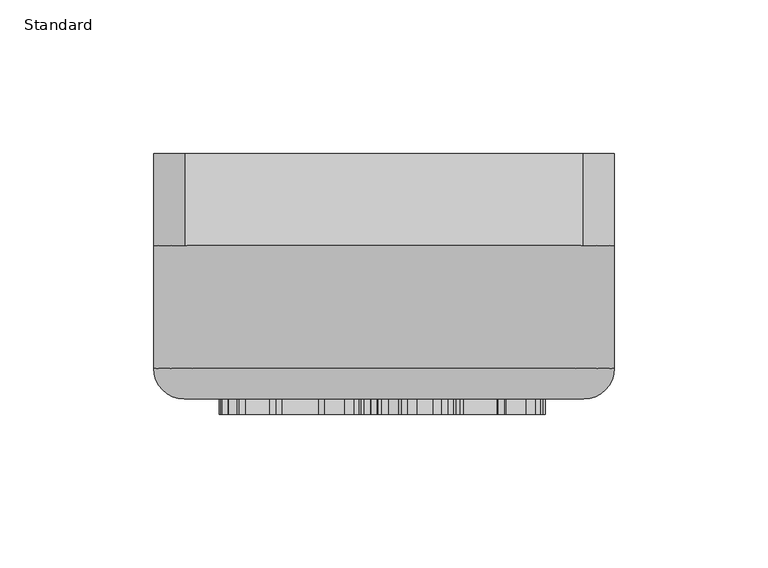
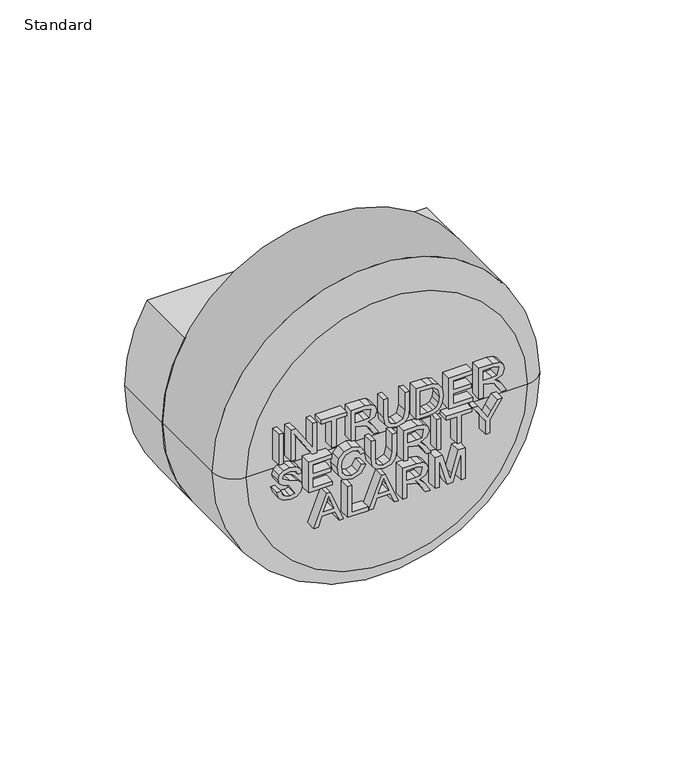
"""IFC4 building model written with IfcOpenShell, lengths in millimetres: proxy geometry, Intruder Security Alarm Sounder : Standard."""

from ifc_helpers import new_model, si_unit, point, frame, origin, origin_2d, place, context, project, spatial, polyline, circle_curve, ellipse_curve, trimmed, segment, composite_curve, outline, extrude, source, transform, mapped, element, save
from ifc_brep_helpers import plane_surface, cylinder_surface, revolved_surface, advanced_brep


def standard_da8f596e(model_context):
    return source(origin(), model_context, "Body", "SolidModel", [
        extrude(outline(polyline([(-50.8099209, -85.0), (-52.6934767, -85.0), (-52.6934767, -80.0), (-50.8099209, -80.0), (-50.8099209, -85.0)])), frame((0.0, 0.0, 4.6605901), z_axis=(0.0, 0.0, 1.0), x_axis=(1.0, 0.0, 0.0)), (0.0, 0.0, 1.0), 15.0684465),
        extrude(outline(polyline([(4.6605901, -47.0428093), (4.6605901, -45.1592535), (16.6020397, -45.1592535), (4.6605901, -37.2865788), (4.6605901, -35.2705855), (19.7290366, -35.2705855), (19.7290366, -37.1541413), (7.7912659, -37.1541413), (19.7290366, -45.026816), (19.7290366, -47.0428093), (4.6605901, -47.0428093)])), frame((0.0, -85.0, 0.0), z_axis=(0.0, 1.0, 0.0), x_axis=(0.0, 0.0, 1.0)), (0.0, 0.0, 1.0), 5.0),
        extrude(outline(polyline([(4.6605901, -28.2072512), (4.6605901, -26.3236953), (17.8454808, -26.3236953), (17.8454808, -21.3793613), (19.7290366, -21.3793613), (19.7290366, -33.1515852), (17.8454808, -33.1515852), (17.8454808, -28.2072512), (4.6605901, -28.2072512)])), frame((0.0, -85.0, 0.0), z_axis=(0.0, 1.0, 0.0), x_axis=(0.0, 0.0, 1.0)), (0.0, 0.0, 1.0), 5.0),
        extrude(outline(polyline([(4.6605901, -19.260361), (4.6605901, -17.3768052), (11.2530355, -17.3768052), (9.8514051, -12.1197715), (7.7839082, -10.7034258), (4.6605901, -8.7426148), (4.6605901, -6.5537169), (8.7440802, -9.0663509), (11.4884799, -11.6635978), (12.8901103, -8.5090097), (15.6050795, -7.4881372), (17.8841084, -8.1043395), (19.322527, -9.7524509), (19.7290366, -12.7672438), (19.7290366, -19.260361), (4.6605901, -19.260361)]), holes=[polyline([(13.1365913, -17.3768052), (17.8454808, -17.3768052), (17.8454808, -12.6863098), (17.1943297, -10.1681575), (13.4033057, -11.0106073), (13.1365913, -13.1608775), (13.1365913, -17.3768052)])]), frame((0.0, -85.0, 0.0), z_axis=(0.0, 1.0, 0.0), x_axis=(0.0, 0.0, 1.0)), (0.0, 0.0, 1.0), 5.0),
        extrude(outline(polyline([(19.7290366, 5.6967535), (11.1022038, 5.6967535), (7.298304, 4.7439392), (6.3087014, 1.5544023), (6.809021, -0.6602474), (8.2308849, -1.9367979), (11.1022038, -2.3083587), (19.7290366, -2.3083587), (19.7290366, -4.1919145), (11.0359851, -4.1919145), (7.2633552, -3.619858), (5.153552, -1.7105504), (4.4251456, 1.7309856), (5.2620772, 5.2258646), (7.4325809, 7.0689534), (11.0359851, 7.5803093), (19.7290366, 7.5803093), (19.7290366, 5.6967535)])), frame((0.0, -85.0, 0.0), z_axis=(0.0, 1.0, 0.0), x_axis=(0.0, 0.0, 1.0)), (0.0, 0.0, 1.0), 5.0),
        extrude(outline(polyline([(4.6605901, 10.876532), (4.6605901, 16.3248644), (4.9181075, 18.7473673), (5.674105, 20.5481497), (7.0407866, 21.9240283), (9.2352027, 22.9540979), (12.2757474, 23.3550893), (15.858918, 22.7627993), (18.434092, 20.9785716), (19.5119862, 18.763922), (19.7290366, 16.0747046), (19.7290366, 10.876532), (4.6605901, 10.876532)]), holes=[polyline([(6.5441459, 12.7600878), (17.8454808, 12.7600878), (17.8454808, 16.0415952), (17.5438176, 18.7124185), (15.8736333, 20.6677113), (12.305178, 21.4715335), (9.4559319, 21.0613451), (7.585252, 19.9153926), (6.8163786, 18.5174411), (6.5441459, 16.0930987), (6.5441459, 12.7600878)])]), frame((0.0, -85.0, 0.0), z_axis=(0.0, 1.0, 0.0), x_axis=(0.0, 0.0, 1.0)), (0.0, 0.0, 1.0), 5.0),
        extrude(outline(polyline([(4.6605901, 25.9449785), (4.6605901, 37.010869), (6.5441459, 37.010869), (6.5441459, 27.8285344), (11.4884799, 27.8285344), (11.4884799, 36.3045355), (13.3720357, 36.3045355), (13.3720357, 27.8285344), (17.8454808, 27.8285344), (17.8454808, 36.7754245), (19.7290366, 36.7754245), (19.7290366, 25.9449785), (4.6605901, 25.9449785)])), frame((0.0, -85.0, 0.0), z_axis=(0.0, 1.0, 0.0), x_axis=(0.0, 0.0, 1.0)), (0.0, 0.0, 1.0), 5.0),
        extrude(outline(polyline([(4.6605901, 39.8362027), (4.6605901, 41.7197585), (11.2530355, 41.7197585), (9.8514051, 46.9767922), (7.7839082, 48.3931379), (4.6605901, 50.3539489), (4.6605901, 52.5428468), (8.7440802, 50.0302128), (11.4884799, 47.4329659), (12.8901103, 50.587554), (15.6050795, 51.6084265), (17.8841084, 50.9922242), (19.322527, 49.3441128), (19.7290366, 46.3293199), (19.7290366, 39.8362027), (4.6605901, 39.8362027)]), holes=[polyline([(13.1365913, 41.7197585), (17.8454808, 41.7197585), (17.8454808, 46.4102539), (17.1943297, 48.9284062), (13.4033057, 48.0859564), (13.1365913, 45.9356862), (13.1365913, 41.7197585)])]), frame((0.0, -85.0, 0.0), z_axis=(0.0, 1.0, 0.0), x_axis=(0.0, 0.0, 1.0)), (0.0, 0.0, 1.0), 5.0),
        extrude(outline(polyline([(-8.4558541, -53.6352547), (-11.3326913, -52.8222354), (-13.23832, -50.6940381), (-13.8710771, -47.3297573), (-13.2843053, -44.4805112), (-11.6398728, -42.5380943), (-9.3865955, -41.8630308), (-7.2565588, -42.4498026), (-5.7298485, -44.2726579), (-4.7843918, -47.6056688), (-2.4262682, -51.2808099), (-0.8627697, -50.4346813), (-0.2152974, -47.7381063), (-0.8701273, -45.0488889), (-2.8051866, -43.9820311), (-2.8051866, -42.0984753), (-0.447063, -42.8452757), (1.1311507, -44.8318385), (1.6682584, -47.8116827), (1.155063, -50.603907), (-0.3495743, -52.5113752), (-2.4814505, -53.1643657), (-4.3539698, -52.636455), (-5.7556002, -51.034329), (-6.6845023, -48.0820759), (-11.6435516, -45.435165), (-11.9875212, -47.4033337), (-11.533187, -49.6621291), (-10.3412493, -51.1446935), (-8.4558541, -51.7516988), (-8.4558541, -53.6352547)])), frame((0.0, -85.0, 0.0), z_axis=(0.0, 1.0, 0.0), x_axis=(0.0, 0.0, 1.0)), (0.0, 0.0, 1.0), 5.0),
        extrude(outline(polyline([(-13.6356326, -39.0376971), (-13.6356326, -27.9718067), (-11.7520768, -27.9718067), (-11.7520768, -37.1541413), (-6.8077427, -37.1541413), (-6.8077427, -28.6781401), (-4.9241869, -28.6781401), (-4.9241869, -37.1541413), (-0.4507419, -37.1541413), (-0.4507419, -28.2072512), (1.4328139, -28.2072512), (1.4328139, -39.0376971), (-13.6356326, -39.0376971)])), frame((0.0, -85.0, 0.0), z_axis=(0.0, 1.0, 0.0), x_axis=(0.0, 0.0, 1.0)), (0.0, 0.0, 1.0), 5.0),
        extrude(outline(polyline([(-8.2792707, -14.5514715), (-11.053101, -16.1499188), (-11.9875212, -19.0322742), (-11.3014213, -21.6313605), (-9.2284063, -23.4008729), (-5.9836871, -23.9692506), (-3.1841051, -23.4891646), (-1.020959, -21.8244985), (-0.2152974, -18.8777638), (-0.9418643, -16.3320203), (-3.2576815, -14.786916), (-2.8088655, -12.9033602), (0.4947149, -15.0315575), (1.6682584, -18.8041874), (0.7614293, -22.4241462), (-1.8928393, -24.9606925), (-5.9873659, -25.8528064), (-10.0156737, -25.0636995), (-12.8814745, -22.764437), (-13.8710771, -18.8446544), (-12.5632566, -14.9009594), (-8.764875, -12.6679157), (-8.2792707, -14.5514715)])), frame((0.0, -85.0, 0.0), z_axis=(0.0, 1.0, 0.0), x_axis=(0.0, 0.0, 1.0)), (0.0, 0.0, 1.0), 5.0),
        extrude(outline(polyline([(1.4328139, -0.1893584), (-7.1940188, -0.1893584), (-10.9979187, -1.1421728), (-11.9875212, -4.3317097), (-11.4872017, -6.5463593), (-10.0653378, -7.8229098), (-7.1940188, -8.1944706), (1.4328139, -8.1944706), (1.4328139, -10.0780264), (-7.2602376, -10.0780264), (-11.0328675, -9.5059699), (-13.1426707, -7.5966624), (-13.8710771, -4.1551263), (-13.0341455, -0.6602474), (-10.8636417, 1.1828414), (-7.2602376, 1.6941974), (1.4328139, 1.6941974), (1.4328139, -0.1893584)])), frame((0.0, -85.0, 0.0), z_axis=(0.0, 1.0, 0.0), x_axis=(0.0, 0.0, 1.0)), (0.0, 0.0, 1.0), 5.0),
        extrude(outline(polyline([(-13.6356326, 4.9904201), (-13.6356326, 6.8739759), (-7.0431872, 6.8739759), (-8.4448176, 12.1310096), (-10.5123144, 13.5473553), (-13.6356326, 15.5081663), (-13.6356326, 17.6970642), (-9.5521424, 15.1844302), (-6.8077427, 12.5871833), (-5.4061123, 15.7417714), (-2.6911432, 16.7626439), (-0.4121143, 16.1464416), (1.0263043, 14.4983303), (1.4328139, 11.4835373), (1.4328139, 4.9904201), (-13.6356326, 4.9904201)]), holes=[polyline([(-5.1596314, 6.8739759), (-0.4507419, 6.8739759), (-0.4507419, 11.5644713), (-1.101893, 14.0826236), (-4.892917, 13.2401738), (-5.1596314, 11.0899036), (-5.1596314, 6.8739759)])]), frame((0.0, -85.0, 0.0), z_axis=(0.0, 1.0, 0.0), x_axis=(0.0, 0.0, 1.0)), (0.0, 0.0, 1.0), 5.0),
        extrude(outline(polyline([(22.1778669, -85.0), (20.2943111, -85.0), (20.2943111, -80.0), (22.1778669, -80.0), (22.1778669, -85.0)])), frame((0.0, 0.0, -13.6356326), z_axis=(0.0, 0.0, 1.0), x_axis=(1.0, 0.0, 0.0)), (0.0, 0.0, 1.0), 15.0684465),
        extrude(outline(polyline([(-13.6356326, 29.7120902), (-13.6356326, 31.595646), (-0.4507419, 31.595646), (-0.4507419, 36.53998), (1.4328139, 36.53998), (1.4328139, 24.7677562), (-0.4507419, 24.7677562), (-0.4507419, 29.7120902), (-13.6356326, 29.7120902)])), frame((0.0, -85.0, 0.0), z_axis=(0.0, 1.0, 0.0), x_axis=(0.0, 0.0, 1.0)), (0.0, 0.0, 1.0), 5.0),
        extrude(outline(polyline([(-13.6356326, 42.8969809), (-13.6356326, 44.7805367), (-7.25288, 44.7805367), (1.4328139, 50.6666486), (1.4328139, 48.4446414), (-3.0369523, 45.5935559), (-5.5716592, 43.9822328), (-3.206178, 42.3745884), (1.4328139, 39.2328762), (1.4328139, 37.010869), (-7.25288, 42.8969809), (-13.6356326, 42.8969809)])), frame((0.0, -85.0, 0.0), z_axis=(0.0, 1.0, 0.0), x_axis=(0.0, 0.0, 1.0)), (0.0, 0.0, 1.0), 5.0),
        extrude(outline(polyline([(-31.9318553, -36.5544936), (-31.9318553, -34.564252), (-27.2229657, -32.8425643), (-27.2229657, -26.636395), (-31.9318553, -24.9110285), (-31.9318553, -22.9207869), (-16.8634087, -28.9356575), (-16.8634087, -30.539623), (-31.9318553, -36.5544936)]), holes=[polyline([(-25.3394099, -32.1509461), (-21.3111021, -30.6757393), (-18.7469645, -29.7376403), (-21.6348382, -28.6818189), (-25.3394099, -27.3243344), (-25.3394099, -32.1509461)])]), frame((0.0, -85.0, 0.0), z_axis=(0.0, 1.0, 0.0), x_axis=(0.0, 0.0, 1.0)), (0.0, 0.0, 1.0), 5.0),
        extrude(outline(polyline([(-31.9318553, -20.9084724), (-31.9318553, -11.4906933), (-30.0482994, -11.4906933), (-30.0482994, -19.0249166), (-16.8634087, -19.0249166), (-16.8634087, -20.9084724), (-31.9318553, -20.9084724)])), frame((0.0, -85.0, 0.0), z_axis=(0.0, 1.0, 0.0), x_axis=(0.0, 0.0, 1.0)), (0.0, 0.0, 1.0), 5.0),
        extrude(outline(polyline([(-31.9318553, -11.1264901), (-31.9318553, -9.1362485), (-27.2229657, -7.4145608), (-27.2229657, -1.2083915), (-31.9318553, 0.516975), (-31.9318553, 2.5072166), (-16.8634087, -3.507654), (-16.8634087, -5.1116195), (-31.9318553, -11.1264901)]), holes=[polyline([(-25.3394099, -6.7229426), (-21.3111021, -5.2477358), (-18.7469645, -4.3096367), (-21.6348382, -3.2538154), (-25.3394099, -1.8963309), (-25.3394099, -6.7229426)])]), frame((0.0, -85.0, 0.0), z_axis=(0.0, 1.0, 0.0), x_axis=(0.0, 0.0, 1.0)), (0.0, 0.0, 1.0), 5.0),
        extrude(outline(polyline([(-31.9318553, 4.5195311), (-31.9318553, 6.403087), (-25.3394099, 6.403087), (-26.7410403, 11.6601207), (-28.8085371, 13.0764663), (-31.9318553, 15.0372774), (-31.9318553, 17.2261753), (-27.8483651, 14.7135412), (-25.1039654, 12.1162943), (-23.702335, 15.2708824), (-20.9873659, 16.291755), (-18.7083369, 15.6755526), (-17.2699183, 14.0274413), (-16.8634087, 11.0126484), (-16.8634087, 4.5195311), (-31.9318553, 4.5195311)]), holes=[polyline([(-23.4558541, 6.403087), (-18.7469645, 6.403087), (-18.7469645, 11.0935824), (-19.3981157, 13.6117347), (-23.1891396, 12.7692849), (-23.4558541, 10.6190146), (-23.4558541, 6.403087)])]), frame((0.0, -85.0, 0.0), z_axis=(0.0, 1.0, 0.0), x_axis=(0.0, 0.0, 1.0)), (0.0, 0.0, 1.0), 5.0),
        extrude(outline(polyline([(-31.9318553, 19.5879777), (-31.9318553, 21.4715335), (-18.7469645, 21.4715335), (-31.9318553, 25.2570392), (-31.9318553, 27.8101403), (-18.7469645, 31.595646), (-31.9318553, 31.595646), (-31.9318553, 33.4792018), (-16.8634087, 33.4792018), (-16.8634087, 30.2381614), (-27.3002209, 27.2068138), (-29.7024904, 26.5335897), (-27.4841619, 25.9118692), (-16.8634087, 22.829018), (-16.8634087, 19.5879777), (-31.9318553, 19.5879777)])), frame((0.0, -85.0, 0.0), z_axis=(0.0, 1.0, 0.0), x_axis=(0.0, 0.0, 1.0)), (0.0, 0.0, 1.0), 5.0),
        extrude(outline(composite_curve([segment(polyline([(38.0, 64.6606526), (38.0, -64.6606526)]), True, "CONTINUOUS"), segment(trimmed(circle_curve(origin_2d(), 75.0), [point((38.0, -64.6606526))], [point((0.0, -75.0))], False, "CARTESIAN"), True, "CONTINUOUS"), segment(trimmed(circle_curve(origin_2d(), 75.0), [point((0.0, -75.0))], [point((-56.0, -49.8898787))], False, "CARTESIAN"), True, "CONTINUOUS"), segment(polyline([(-56.0, -49.8898787), (-56.0, 49.8898787)]), True, "CONTINUOUS"), segment(trimmed(circle_curve(origin_2d(), 75.0), [point((-56.0, 49.8898787))], [point((0.0, 75.0))], False, "CARTESIAN"), True, "CONTINUOUS"), segment(trimmed(circle_curve(origin_2d(), 75.0), [point((0.0, 75.0))], [point((38.0, 64.6606526))], False, "CARTESIAN"), True, "CONTINUOUS")], self_intersect=False)), frame((0.0, -30.0, 0.0), z_axis=(0.0, 1.0, 0.0), x_axis=(0.0, 0.0, 1.0)), (0.0, 0.0, 1.0), 30.0),
        advanced_brep(
        [(-65.0, -80.0, 0.0), (65.0, -80.0, 0.0), (0.0, -80.0, 0.0), (-75.0, -70.0, 0.0), (75.0, -70.0, 0.0), (-75.0, -30.0, 0.0), (75.0, -30.0, 0.0), (0.0, -30.0, 0.0)],
        [
            (0, 1, circle_curve(frame((0.0, -80.0, 0.0), z_axis=(0.0, -1.0, 0.0), x_axis=(1.0, 0.0, 0.0)), 65.0)),
            (1, 2),
            (2, 0),
            (1, 0, circle_curve(frame((0.0, -80.0, 0.0), z_axis=(0.0, -1.0, 0.0), x_axis=(1.0, 0.0, 0.0)), 65.0)),
            (3, 4, circle_curve(frame((0.0, -70.0, 0.0), z_axis=(0.0, -1.0, 0.0), x_axis=(1.0, 0.0, 0.0)), 75.0)),
            (4, 1, circle_curve(frame((65.0, -70.0, 0.0), z_axis=(0.0, 0.0, -1.0), x_axis=(-1.0, 0.0, 0.0)), 10.0)),
            (0, 3, circle_curve(frame((-65.0, -70.0, 0.0), z_axis=(0.0, 0.0, -1.0), x_axis=(1.0, 0.0, 0.0)), 10.0)),
            (4, 3, circle_curve(frame((0.0, -70.0, 0.0), z_axis=(0.0, -1.0, 0.0), x_axis=(1.0, 0.0, 0.0)), 75.0)),
            (5, 6, circle_curve(frame((0.0, -30.0, 0.0), z_axis=(0.0, -1.0, 0.0), x_axis=(1.0, 0.0, 0.0)), 75.0)),
            (6, 4),
            (3, 5),
            (6, 5, circle_curve(frame((0.0, -30.0, 0.0), z_axis=(0.0, -1.0, 0.0), x_axis=(1.0, 0.0, 0.0)), 75.0)),
            (7, 6),
            (5, 7),
        ],
        [
            plane_surface(frame((0.0, -80.0, 0.0), z_axis=(0.0, -1.0, 0.0), x_axis=(1.0, 0.0, 0.0))),
            revolved_surface(trimmed(ellipse_curve(frame((65.0, -70.0, 0.0), z_axis=(0.0, 0.0, 1.0), x_axis=(-1.0, 0.0, 0.0)), 10.0, 10.0), [point((65.0, -80.0, 0.0))], [point((75.0, -70.0, 0.0))], True, "CARTESIAN"), (0.0, 0.0, 0.0), (0.0, 1.0, 0.0)),
            cylinder_surface(frame((0.0, 0.0, 0.0), z_axis=(0.0, 1.0, 0.0), x_axis=(1.0, 0.0, 0.0)), 75.0),
            plane_surface(frame((0.0, -30.0, 0.0), z_axis=(0.0, 1.0, 0.0), x_axis=(1.0, 0.0, 0.0))),
        ],
        [
            (0, [[1, 2, 3]]),
            (0, [[4, -3, -2]]),
            (1, [[5, 6, -1, 7]]),
            (1, [[8, -7, -4, -6]]),
            (2, [[9, 10, -5, 11]]),
            (2, [[12, -11, -8, -10]]),
            (3, [[13, -9, 14]]),
            (3, [[-14, -12, -13]]),
        ],
    ),
    ])


if __name__ == "__main__":
    model = new_model("IFC4")
    model_context = context("Model", 3, world=origin())
    ifc_project = project(units=[si_unit("LENGTHUNIT", "METRE", prefix="MILLI")], contexts=[model_context])
    site = spatial("IfcSite", under=ifc_project)
    building = spatial("IfcBuilding", under=site)
    placement = place(None, origin())
    standard_shape = standard_da8f596e(model_context)
    element("IfcBuildingElementProxy", 1, Name="Intruder Security Alarm Sounder : Standard", ObjectType="Intruder Security Alarm Sounder : Standard", at=placement, inside=building, context=model_context, shape_type="MappedRepresentation", body=[
        mapped(standard_shape, transform((0.0, 0.0, 0.0), x_axis=(1.0, 0.0, 0.0), y_axis=(0.0, 1.0, 0.0), z_axis=(0.0, 0.0, 1.0))),
    ])
    save(model, "model.ifc")

# Revit data of these elements
# Type "Intruder Security Alarm Sounder : Standard"
#   Type Mark = "Intruder Security Alarm Sounder"
#   Classification.OmniClass.21.Number = "21-04 70 50"
#   Classification.MasterFormat.Description = "Electronic Detection and Alarm"
#   Classification.OmniClass.21.Description = "Detection and Alarm"
#   Classification.UniFormat.II.Description = "Detection and Alarm"
#   Classification.MasterFormat.Number = "28 30 00"
#   Classification.OmniClass.23.Number = "23-29 11 23 15"
#   Classification.OmniClass.23.Description = "Intrusion Detection Microwave Alarms"
#   Classification.UniFormat.II.Number = "D7050"
#   COBie.Type.CreatedBy = "info@mma.ie"
#   COBie.Type.CreatedOn = "2017-07-26T09:25:07"
#   COBie.Type.Name = "Intruder Security Alarm Sounder"
#   COBie.Type.Category = "23-29 11 23 15 : Intrusion Detection Microwave Alarms"
#   COBie.Type.Description = "Intruder Security Alarm Sounder_Intruder Security Alarm Sounder"
#   COBie.Type.AssetType = "Fixed"
#   COBie.Type.Manufacturer = ""
#   COBie.Type.ModelNumber = ""
#   Standard = ""
#   SounderType = ""
#   SounderCutOffTimeMaximum = ""
#   PowerSupply = ""
#   Mounting = ""
#   Keynote = "28 01 30.51.A"
#   IntegralBeacon = ""
#   IngressProtectionStandard = ""
#   I.A. Audio Level = "75dB"
#   DirectionalOutputAt1MMinimum = ""
#   COBie.Type.ReplacementCost = 0
#   UsageCurrent = 0
#   SounderRadius = 75 mm
#   SounderDepth = 50 mm
#   PlanSymbolOffset [instance default] = 250 mm
#   PlanSymbolAlignment [instance default] = 0 mm
#   PhaseAngle = 0.00°
#   NominalVoltage = 0
#   NominalLength = 150 mm
#   NominalHeight = 80 mm
#   NominalFrequencyRange = 0
#   NominalCurrent = 0
#   I.A. Diameter = 150 mm
#   I.A. Depth = 50 mm
#   BaseLevelOffset = 0 mm
#   BackingCaseDepth = 30 mm
#   COBie.Type = yes
#   PlanSymbolVisibility [instance default] = yes
#   PlanObjectVisibility [instance default] = yes
#   NumberOfPoles = 0
#   HasProtectiveEarth = yes
#   URL = ""
#   Type Comments = ""
#   Model = ""
#   Manufacturer = ""
#   Description = (empty or 0)
#   Default Elevation = 0
#   Assembly Code = ""
# Element 1 (IfcBuildingElementProxy, "Intruder Security Alarm Sounder : Standard")
#   Materials on its faces: "nbl_ConceptWhite"
# Materials
#   "nbl_ConceptWhite": class "Generic", colour RGB 255 255 255, transparency 0, Cost = 0
